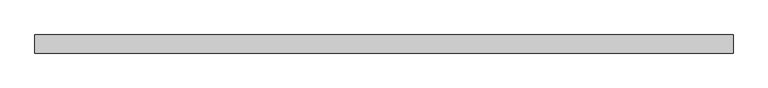
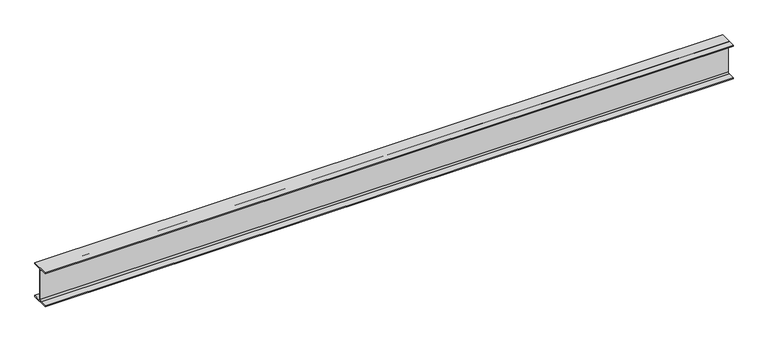
"""IFC4 building model written with IfcOpenShell, lengths in millimetres: beam geometry, Steel Framing_H_KS : H_SB_AR_S02_H-300x150x6.5x9_SRB3."""

from ifc_helpers import new_model, si_unit, point, frame, frame_2d, origin, place, context, project, spatial, polyline, circle_curve, trimmed, segment, composite_curve, outline, extrude, source, transform, mapped, element, save


def beam_98be4253(model_context):
    return source(origin(), model_context, "Body", "SweptSolid", [
        extrude(outline(composite_curve([segment(polyline([(75.0, -141.0), (75.0, -150.0), (-75.0, -150.0), (-75.0, -141.0), (-16.25, -141.0)]), True, "CONTINUOUS"), segment(trimmed(circle_curve(frame_2d((-16.25, -128.0)), 13.0), [point((-16.25, -141.0))], [point((-3.25, -128.0))], True, "CARTESIAN"), True, "CONTINUOUS"), segment(polyline([(-3.25, -128.0), (-3.25, 128.0)]), True, "CONTINUOUS"), segment(trimmed(circle_curve(frame_2d((-16.25, 128.0)), 13.0), [point((-3.25, 128.0))], [point((-16.25, 141.0))], True, "CARTESIAN"), True, "CONTINUOUS"), segment(polyline([(-16.25, 141.0), (-75.0, 141.0), (-75.0, 150.0), (75.0, 150.0), (75.0, 141.0), (16.25, 141.0)]), True, "CONTINUOUS"), segment(trimmed(circle_curve(frame_2d((16.25, 128.0)), 13.0), [point((16.25, 141.0))], [point((3.25, 128.0))], True, "CARTESIAN"), True, "CONTINUOUS"), segment(polyline([(3.25, 128.0), (3.25, -128.0)]), True, "CONTINUOUS"), segment(trimmed(circle_curve(frame_2d((16.25, -128.0)), 13.0), [point((3.25, -128.0))], [point((16.25, -141.0))], True, "CARTESIAN"), True, "CONTINUOUS"), segment(polyline([(16.25, -141.0), (75.0, -141.0)]), True, "CONTINUOUS")], self_intersect=False)), frame((-2887.3, 0.0, 0.0), z_axis=(1.0, 0.0, 0.0), x_axis=(0.0, 1.0, 0.0)), (0.0, 0.0, 1.0), 5774.6),
    ])


if __name__ == "__main__":
    model = new_model("IFC4")
    model_context = context("Model", 3, world=origin())
    ifc_project = project(units=[si_unit("LENGTHUNIT", "METRE", prefix="MILLI")], contexts=[model_context])
    site = spatial("IfcSite", under=ifc_project)
    building = spatial("IfcBuilding", under=site)
    placement = place(None, origin())
    beam_shape = beam_98be4253(model_context)
    element("IfcBeam", 1, ObjectType="Steel Framing_H_KS : H_SB_AR_S02_H-300x150x6.5x9_SRB3", at=placement, inside=building, context=model_context, shape_type="MappedRepresentation", body=[
        mapped(beam_shape, transform((0.0, 0.0, 0.0), x_axis=(1.0, 0.0, 0.0), y_axis=(0.0, 1.0, 0.0), z_axis=(0.0, 0.0, 1.0))),
    ])
    save(model, "model.ifc")

# Revit data of these elements
# Type "Steel Framing_H_KS : H_SB_AR_S02_H-300x150x6.5x9_SRB3"
#   Type Comments = "MAIN"
#   Type Mark = "SRB3"
#   H_SectionID = "H-300x150x6.5x9"
#   H_Ratio for Additional Steel Plate = 0.2
#   Width = 15.0 cm
#   Web Thickness = 0.65 cm
#   Web Fillet = 1.3 cm
#   Warping Constant = 107000.0 cm⁶
#   Torsional Moment of Inertia = 9.9539 cm⁴
#   Section Area = 46.78 cm²
#   Plastic Modulus weak axis = 105.0 cm³
#   Plastic Modulus strong axis = 542.0 cm³
#   Perimeter = 1.17 m²/m
#   Nominal Weight = 36.70 kgf/m
#   Moment of Inertia weak axis = 508.00 cm⁴
#   Moment of Inertia strong axis = 7210.00 cm⁴
#   Height = 30.0 cm
#   Flange Thickness = 0.9 cm
#   Elastic Modulus weak axis = 67.7 cm³
#   Elastic Modulus strong axis = 481.0 cm³
#   Centroid Vertical = 15.0 cm
#   Centroid Horizontal = 7.5 cm
#   Bolt Spacing = 8.89 cm
#   Length [instance default] = 1500 mm
#   Structural Material [instance default] = Steel, 45-345
#   Section Name Key = ""
#   Assembly Code = ""
# Element 1 (IfcBeam, "Steel Framing_H_KS : H_SB_AR_S02_H-300x150x6.5x9_SRB3")
#   Materials on its faces: "Steel, 45-345"
# Materials
#   "Steel, 45-345": class "Metal", colour RGB 189 187 185, transparency 0, Description = "Steel 345 MPa", Cost = 0
